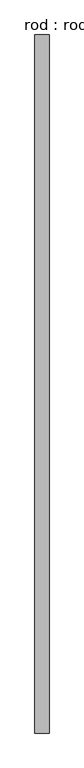
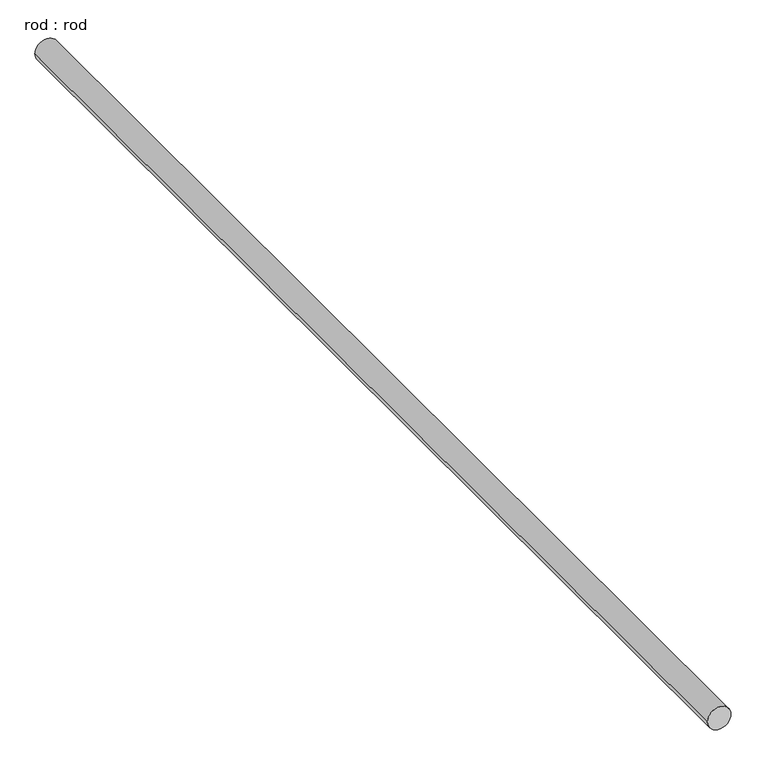
"""IFC4 building model written with IfcOpenShell, lengths in millimetres: proxy geometry, rod : rod."""

from ifc_helpers import new_model, si_unit, point, frame, frame_2d, origin, place, context, project, spatial, circle_curve, trimmed, segment, composite_curve, outline, extrude, source, transform, mapped, element, save


def rod_rod_75b11795(model_context):
    return source(origin(), model_context, "Body", "SweptSolid", [
        extrude(outline(composite_curve([segment(trimmed(circle_curve(frame_2d((0.0108462, 0.0)), 200.0), [point((0.0108462, 200.0))], [point((0.0108462, -200.0))], False, "CARTESIAN"), True, "CONTINUOUS"), segment(trimmed(circle_curve(frame_2d((0.0108462, 0.0)), 200.0), [point((0.0108462, -200.0))], [point((0.0108462, 200.0))], False, "CARTESIAN"), True, "CONTINUOUS")], self_intersect=False)), frame((0.0, -5778.2721726, 0.0), z_axis=(0.0, 1.0, 0.0), x_axis=(0.0, 0.0, 1.0)), (0.0, 0.0, 1.0), 19742.0015759),
    ])


if __name__ == "__main__":
    model = new_model("IFC4")
    model_context = context("Model", 3, world=origin())
    ifc_project = project(units=[si_unit("LENGTHUNIT", "METRE", prefix="MILLI")], contexts=[model_context])
    site = spatial("IfcSite", under=ifc_project)
    building = spatial("IfcBuilding", under=site)
    placement = place(None, origin())
    rod_rod_shape = rod_rod_75b11795(model_context)
    element("IfcBuildingElementProxy", 1, Name="rod : rod", ObjectType="rod : rod", at=placement, inside=building, context=model_context, shape_type="MappedRepresentation", body=[
        mapped(rod_rod_shape, transform((0.0, 0.0, 0.0), x_axis=(1.0, 0.0, 0.0), y_axis=(0.0, 1.0, 0.0), z_axis=(0.0, 0.0, 1.0))),
    ])
    save(model, "model.ifc")

# Revit data of these elements
# Type "rod : rod"
#   Default Elevation = 0
